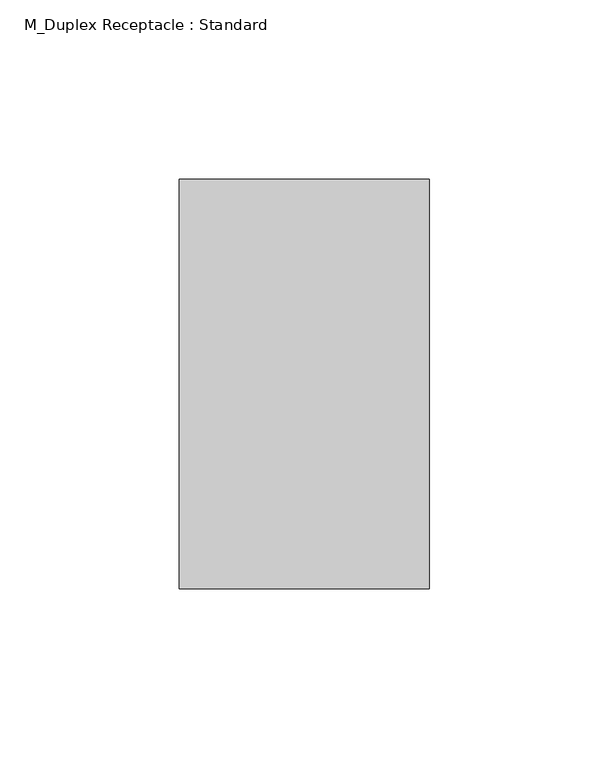
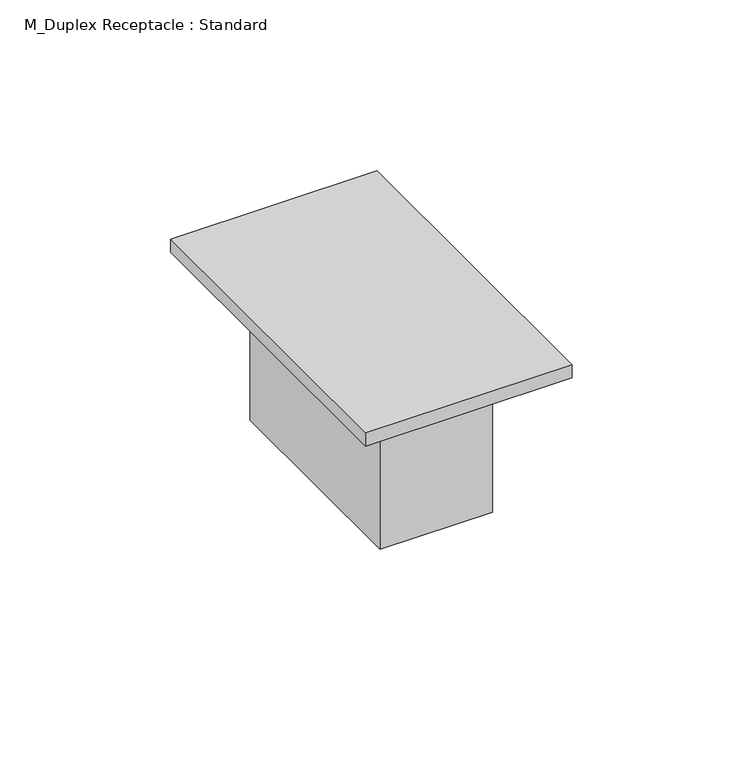
"""IFC4 building model written with IfcOpenShell, lengths in millimetres: proxy geometry, M_Duplex Receptacle : Standard."""

from ifc_helpers import new_model, si_unit, frame, origin, origin_with_axes, place, context, project, spatial, polyline, outline, extrude, source, transform, mapped, element, save


def m_duplex_receptacle_standard_367a9a66(model_context):
    return source(origin(), model_context, "Body", "SweptSolid", [
        extrude(outline(polyline([(34.925, 57.15), (34.925, -57.15), (-34.925, -57.15), (-34.925, 57.15), (34.925, 57.15)])), origin_with_axes(), (0.0, 0.0, 1.0), 4.7625),
        extrude(outline(polyline([(19.05, 38.1), (19.05, -38.1), (-19.05, -38.1), (-19.05, 38.1), (19.05, 38.1)])), frame((0.0, 0.0, -53.975), z_axis=(0.0, 0.0, 1.0), x_axis=(1.0, 0.0, 0.0)), (0.0, 0.0, 1.0), 53.975),
    ])


if __name__ == "__main__":
    model = new_model("IFC4")
    model_context = context("Model", 3, world=origin())
    ifc_project = project(units=[si_unit("LENGTHUNIT", "METRE", prefix="MILLI")], contexts=[model_context])
    site = spatial("IfcSite", under=ifc_project)
    building = spatial("IfcBuilding", under=site)
    placement = place(None, origin())
    m_duplex_receptacle_standard_shape = m_duplex_receptacle_standard_367a9a66(model_context)
    element("IfcBuildingElementProxy", 1, Name="M_Duplex Receptacle : Standard", ObjectType="M_Duplex Receptacle : Standard", at=placement, inside=building, context=model_context, shape_type="MappedRepresentation", body=[
        mapped(m_duplex_receptacle_standard_shape, transform((0.0, 0.0, 0.0), x_axis=(1.0, 0.0, 0.0), y_axis=(0.0, 1.0, 0.0), z_axis=(0.0, 0.0, 1.0))),
    ])
    save(model, "model.ifc")

# Revit data of these elements
# Type "M_Duplex Receptacle : Standard"
#   Label = ""
#   Switch Voltage = 120 V
#   Load = 180 VA
#   Default Elevation = 0.46 m
#   Load Classification = Receptacle
